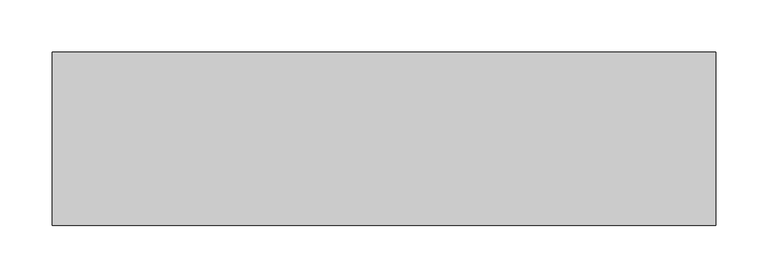
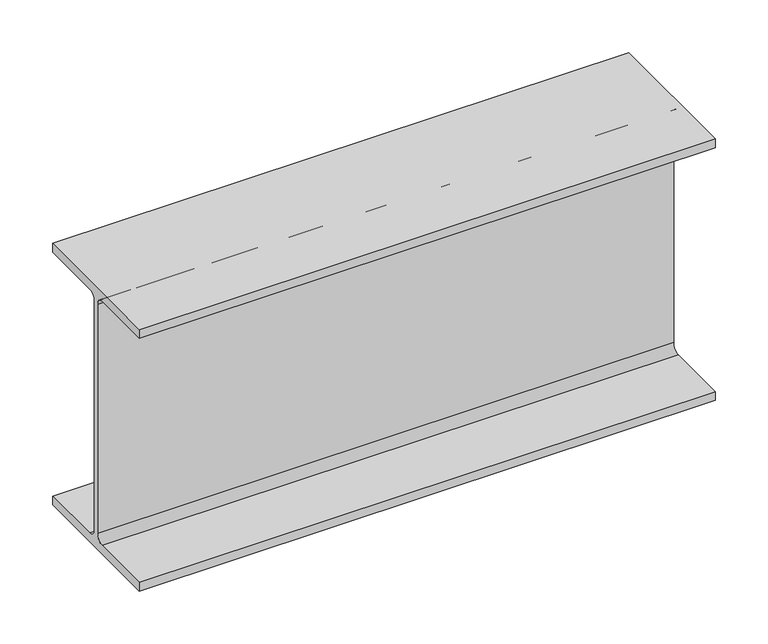
"""IFC4 building model written with IfcOpenShell, lengths in millimetres: beam geometry, Old_Steel Beam_H-KSD3502 : H_SB_ASB_H-300×150x6.5x9."""

from ifc_helpers import new_model, si_unit, point, frame, frame_2d, origin, place, context, project, spatial, polyline, circle_curve, trimmed, segment, composite_curve, outline, extrude, source, transform, mapped, element, save


def beam_590130a8(model_context):
    return source(origin(), model_context, "Body", "SweptSolid", [
        extrude(outline(composite_curve([segment(polyline([(82.5, -141.5), (82.5, -151.7), (-82.5, -151.7), (-82.5, -141.5), (-11.9, -141.5)]), True, "CONTINUOUS"), segment(trimmed(circle_curve(frame_2d((-11.9, -132.6)), 8.9), [point((-11.9, -141.5))], [point((-3.0, -132.6))], True, "CARTESIAN"), True, "CONTINUOUS"), segment(polyline([(-3.0, -132.6), (-3.0, 132.6)]), True, "CONTINUOUS"), segment(trimmed(circle_curve(frame_2d((-11.9, 132.6)), 8.9), [point((-3.0, 132.6))], [point((-11.9, 141.5))], True, "CARTESIAN"), True, "CONTINUOUS"), segment(polyline([(-11.9, 141.5), (-82.5, 141.5), (-82.5, 151.7), (82.5, 151.7), (82.5, 141.5), (11.9, 141.5)]), True, "CONTINUOUS"), segment(trimmed(circle_curve(frame_2d((11.9, 132.6)), 8.9), [point((11.9, 141.5))], [point((3.0, 132.6))], True, "CARTESIAN"), True, "CONTINUOUS"), segment(polyline([(3.0, 132.6), (3.0, -132.6)]), True, "CONTINUOUS"), segment(trimmed(circle_curve(frame_2d((11.9, -132.6)), 8.9), [point((3.0, -132.6))], [point((11.9, -141.5))], True, "CARTESIAN"), True, "CONTINUOUS"), segment(polyline([(11.9, -141.5), (82.5, -141.5)]), True, "CONTINUOUS")], self_intersect=False)), frame((-349.8, 0.0, 0.0), z_axis=(1.0, 0.0, 0.0), x_axis=(0.0, 1.0, 0.0)), (0.0, 0.0, 1.0), 632.1),
    ])


if __name__ == "__main__":
    model = new_model("IFC4")
    model_context = context("Model", 3, world=origin())
    ifc_project = project(units=[si_unit("LENGTHUNIT", "METRE", prefix="MILLI")], contexts=[model_context])
    site = spatial("IfcSite", under=ifc_project)
    building = spatial("IfcBuilding", under=site)
    placement = place(None, origin())
    beam_shape = beam_590130a8(model_context)
    element("IfcBeam", 1, ObjectType="Old_Steel Beam_H-KSD3502 : H_SB_ASB_H-300×150x6.5x9", at=placement, inside=building, context=model_context, shape_type="MappedRepresentation", body=[
        mapped(beam_shape, transform((0.0, 0.0, 0.0), x_axis=(1.0, 0.0, 0.0), y_axis=(0.0, 1.0, 0.0), z_axis=(0.0, 0.0, 1.0))),
    ])
    save(model, "model.ifc")

# Revit data of these elements
# Type "Old_Steel Beam_H-KSD3502 : H_SB_ASB_H-300×150x6.5x9"
#   Width = 15.0 cm
#   Web Thickness = 0.65 cm
#   Web Fillet = 1.3 cm
#   Warping Constant = 107174.0 cm⁶
#   Torsional Moment of Inertia = 9.9539 cm⁴
#   Torsional Modulus = 1.0 cm³
#   Section Area = 46.78 cm²
#   Plastic Modulus weak axis = 105.0 cm³
#   Plastic Modulus strong axis = 542.0 cm³
#   Perimeter = 1.17 m²/m
#   Nominal Weight = 36.70 kgf/m
#   Moment of Inertia weak axis = 508.00 cm⁴
#   Moment of Inertia strong axis = 7210.00 cm⁴
#   Height = 30.0 cm
#   Flange Thickness = 0.9 cm
#   Elastic Modulus weak axis = 67.7 cm³
#   Elastic Modulus strong axis = 481.0 cm³
#   Centroid Vertical = 15.0 cm
#   Centroid Horizontal = 7.5 cm
#   Length [instance default] = 1.5240 m
#   Structural Material [instance default] = Steel, 45-345
#   Assembly Code = ""
# Element 1 (IfcBeam, "Old_Steel Beam_H-KSD3502 : H_SB_ASB_H-300×150x6.5x9")
#   Structural Material = none
# Materials
#   "Steel, 45-345": class "Metal", colour RGB 189 187 185, transparency 0, Description = "Steel 345 MPa", Cost = 0
